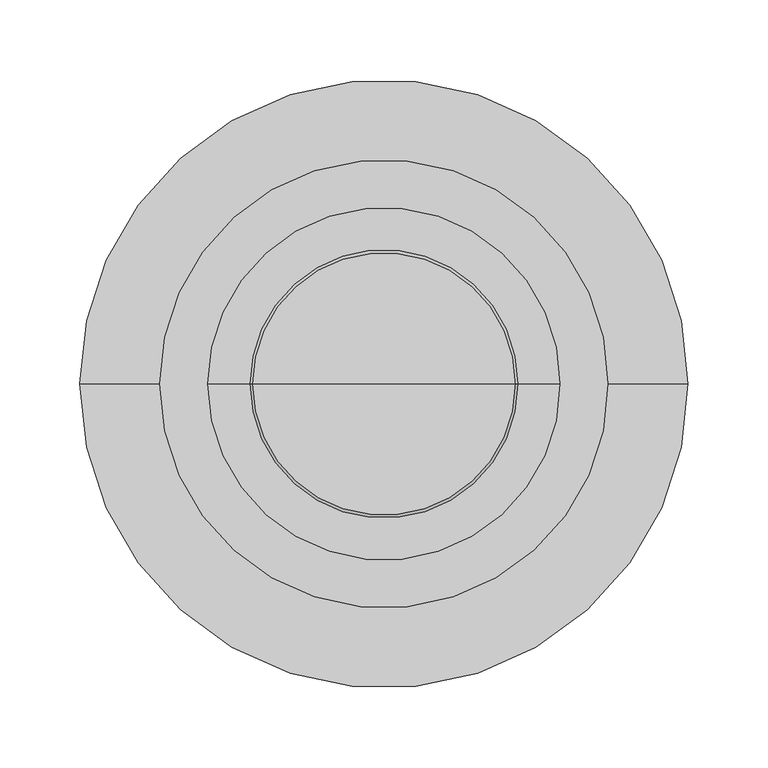
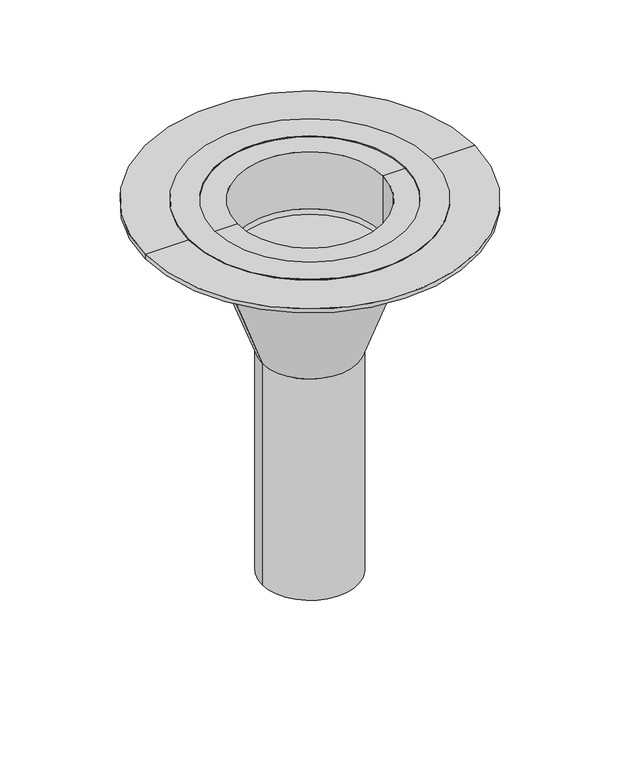
"""IFC4 building model written with IfcOpenShell, lengths in millimetres: proxy geometry, TN_Воронка с обжимным фланцем : Воронка с обжимным металлическим фланцем без обогрева Ø110х450мм."""

from ifc_helpers import new_model, si_unit, point, frame, origin, origin_with_axes, origin_2d, place, context, project, spatial, polyline, circle_curve, trimmed, segment, composite_curve, outline, extrude, source, transform, mapped, element, save
from ifc_brep_helpers import plane_surface, cylinder_surface, revolved_surface, advanced_brep


def specialty_equipment_f296e0ad(model_context):
    return source(origin(), model_context, "Body", "SolidModel", [
        extrude(outline(composite_curve([segment(trimmed(circle_curve(origin_2d(), 140.0), [point((-140.0, 0.0))], [point((140.0, 0.0))], False, "CARTESIAN"), True, "CONTINUOUS"), segment(trimmed(circle_curve(origin_2d(), 140.0), [point((140.0, 0.0))], [point((-140.0, 0.0))], False, "CARTESIAN"), True, "CONTINUOUS")], self_intersect=False), holes=[composite_curve([segment(trimmed(circle_curve(origin_2d(), 110.0556416), [point((-110.0556416, 0.0))], [point((110.0556416, 0.0))], True, "CARTESIAN"), True, "CONTINUOUS"), segment(trimmed(circle_curve(origin_2d(), 110.0556416), [point((110.0556416, 0.0))], [point((-110.0556416, 0.0))], True, "CARTESIAN"), True, "CONTINUOUS")], self_intersect=False)]), origin_with_axes(), (0.0, 0.0, 1.0), 1.0),
        advanced_brep(
        [(0.0, 0.0, -450.0), (-55.0, 0.0, -450.0), (55.0, 0.0, -450.0), (190.0, 0.0, 0.0), (-190.0, 0.0, 0.0), (-83.890873, 0.0, 0.0), (83.890873, 0.0, 0.0), (190.0, 0.0, -5.0), (-190.0, 0.0, -5.0), (93.890873, 0.0, -5.0), (-93.890873, 0.0, -5.0), (55.0, 0.0, -179.9935725), (-55.0, 0.0, -179.9935725), (-93.890873, 0.0, -71.109127), (93.890873, 0.0, -71.109127), (81.9669914, 0.0, -74.7632135), (-81.9669914, 0.0, -74.7632135), (0.0, 0.0, -74.7632135), (83.890873, 0.0, -69.3768397), (-83.890873, 0.0, -69.3768397)],
        [
            (0, 1),
            (1, 2, circle_curve(frame((0.0, 0.0, -450.0), z_axis=(0.0, 0.0, -1.0), x_axis=(-1.0, 0.0, 0.0)), 55.0)),
            (2, 0),
            (2, 1, circle_curve(frame((0.0, 0.0, -450.0), z_axis=(0.0, 0.0, -1.0), x_axis=(-1.0, 0.0, 0.0)), 55.0)),
            (3, 4, circle_curve(frame((0.0, 0.0, 0.0), z_axis=(0.0, 0.0, 1.0), x_axis=(-1.0, 0.0, 0.0)), 190.0)),
            (4, 5),
            (5, 6, circle_curve(frame((0.0, 0.0, 0.0), z_axis=(0.0, 0.0, -1.0), x_axis=(-1.0, 0.0, 0.0)), 83.890873)),
            (6, 3),
            (4, 3, circle_curve(frame((0.0, 0.0, 0.0), z_axis=(0.0, 0.0, 1.0), x_axis=(-1.0, 0.0, 0.0)), 190.0)),
            (6, 5, circle_curve(frame((0.0, 0.0, 0.0), z_axis=(0.0, 0.0, -1.0), x_axis=(-1.0, 0.0, 0.0)), 83.890873)),
            (7, 8, circle_curve(frame((0.0, 0.0, -5.0), z_axis=(0.0, 0.0, 1.0), x_axis=(-1.0, 0.0, 0.0)), 190.0)),
            (8, 4),
            (3, 7),
            (8, 7, circle_curve(frame((0.0, 0.0, -5.0), z_axis=(0.0, 0.0, 1.0), x_axis=(-1.0, 0.0, 0.0)), 190.0)),
            (9, 10, circle_curve(frame((0.0, 0.0, -5.0), z_axis=(0.0, 0.0, 1.0), x_axis=(-1.0, 0.0, 0.0)), 93.890873)),
            (10, 8),
            (7, 9),
            (10, 9, circle_curve(frame((0.0, 0.0, -5.0), z_axis=(0.0, 0.0, 1.0), x_axis=(-1.0, 0.0, 0.0)), 93.890873)),
            (11, 12, circle_curve(frame((0.0, 0.0, -179.9935725), z_axis=(0.0, 0.0, 1.0), x_axis=(-1.0, 0.0, 0.0)), 55.0)),
            (12, 13),
            (13, 14, circle_curve(frame((0.0, 0.0, -71.109127), z_axis=(0.0, 0.0, -1.0), x_axis=(-1.0, 0.0, 0.0)), 93.890873)),
            (14, 11),
            (12, 11, circle_curve(frame((0.0, 0.0, -179.9935725), z_axis=(0.0, 0.0, 1.0), x_axis=(-1.0, 0.0, 0.0)), 55.0)),
            (14, 13, circle_curve(frame((0.0, 0.0, -71.109127), z_axis=(0.0, 0.0, -1.0), x_axis=(-1.0, 0.0, 0.0)), 93.890873)),
            (1, 12),
            (11, 2),
            (15, 16, circle_curve(frame((0.0, 0.0, -74.7632135), z_axis=(0.0, 0.0, 1.0), x_axis=(-1.0, 0.0, 0.0)), 81.9669914)),
            (16, 17),
            (17, 15),
            (16, 15, circle_curve(frame((0.0, 0.0, -74.7632135), z_axis=(0.0, 0.0, 1.0), x_axis=(-1.0, 0.0, 0.0)), 81.9669914)),
            (18, 19, circle_curve(frame((0.0, 0.0, -69.3768397), z_axis=(0.0, 0.0, 1.0), x_axis=(-1.0, 0.0, 0.0)), 83.890873)),
            (19, 16),
            (15, 18),
            (19, 18, circle_curve(frame((0.0, 0.0, -69.3768397), z_axis=(0.0, 0.0, 1.0), x_axis=(-1.0, 0.0, 0.0)), 83.890873)),
            (5, 19),
            (18, 6),
            (13, 10),
            (9, 14),
        ],
        [
            plane_surface(frame((0.0, 0.0, -450.0), z_axis=(0.0, 0.0, -1.0), x_axis=(-1.0, 0.0, 0.0))),
            plane_surface(frame((0.0, 0.0, 0.0), z_axis=(0.0, 0.0, 1.0), x_axis=(-1.0, 0.0, 0.0))),
            cylinder_surface(frame((0.0, 0.0, 0.0), z_axis=(0.0, 0.0, -1.0), x_axis=(-1.0, 0.0, 0.0)), 190.0),
            plane_surface(frame((0.0, 0.0, -5.0), z_axis=(0.0, 0.0, -1.0), x_axis=(-1.0, 0.0, 0.0))),
            revolved_surface(polyline([(-93.890873, 0.0, -71.109127), (-55.0, 0.0, -179.9935725)]), (0.0, 0.0, 0.0), (0.0, 0.0, -1.0)),
            cylinder_surface(frame((0.0, 0.0, 0.0), z_axis=(0.0, 0.0, -1.0), x_axis=(-1.0, 0.0, 0.0)), 55.0),
            plane_surface(frame((0.0, 0.0, -74.7632135), z_axis=(0.0, 0.0, 1.0), x_axis=(-1.0, 0.0, 0.0))),
            revolved_surface(polyline([(-81.9669914, 0.0, -74.7632135), (-83.890873, 0.0, -69.3768397)]), (0.0, 0.0, 0.0), (0.0, 0.0, -1.0)),
            revolved_surface(polyline([(-83.890873, 0.0, -69.3768397), (-83.890873, 0.0, 0.0)]), (0.0, 0.0, 0.0), (0.0, 0.0, -1.0)),
            cylinder_surface(frame((0.0, 0.0, 0.0), z_axis=(0.0, 0.0, -1.0), x_axis=(-1.0, 0.0, 0.0)), 93.890873),
        ],
        [
            (0, [[1, 2, 3]]),
            (0, [[-3, 4, -1]]),
            (1, [[5, 6, 7, 8]]),
            (1, [[9, -8, 10, -6]]),
            (2, [[11, 12, -5, 13]]),
            (2, [[14, -13, -9, -12]]),
            (3, [[15, 16, -11, 17]]),
            (3, [[18, -17, -14, -16]]),
            (4, [[19, 20, 21, 22]]),
            (4, [[23, -22, 24, -20]]),
            (5, [[-2, 25, -19, 26]]),
            (5, [[-4, -26, -23, -25]]),
            (6, [[27, 28, 29]]),
            (6, [[30, -29, -28]]),
            (7, [[31, 32, -27, 33]]),
            (7, [[34, -33, -30, -32]]),
            (8, [[-7, 35, -31, 36]]),
            (8, [[-10, -36, -34, -35]]),
            (9, [[-21, 37, -15, 38]]),
            (9, [[-24, -38, -18, -37]]),
        ],
    ),
    ])


if __name__ == "__main__":
    model = new_model("IFC4")
    model_context = context("Model", 3, world=origin())
    ifc_project = project(units=[si_unit("LENGTHUNIT", "METRE", prefix="MILLI")], contexts=[model_context])
    site = spatial("IfcSite", under=ifc_project)
    building = spatial("IfcBuilding", under=site)
    placement = place(None, origin())
    specialty_equipment_shape = specialty_equipment_f296e0ad(model_context)
    element("IfcBuildingElementProxy", 1, Name="TN_Воронка с обжимным фланцем : Воронка с обжимным металлическим фланцем без обогрева Ø110х450мм", ObjectType="TN_Воронка с обжимным фланцем : Воронка с обжимным металлическим фланцем без обогрева Ø110х450мм", at=placement, inside=building, context=model_context, shape_type="MappedRepresentation", body=[
        mapped(specialty_equipment_shape, transform((0.0, 0.0, 0.0), x_axis=(1.0, 0.0, 0.0), y_axis=(0.0, 1.0, 0.0), z_axis=(0.0, 0.0, 1.0))),
    ])
    save(model, "model.ifc")

# Revit data of these elements
# Type "TN_Воронка с обжимным фланцем : Воронка с обжимным металлическим фланцем без обогрева Ø110х450мм"
#   ADSK_Группирование = "Комплектующие и воронки"
#   Description = "Кровельная воронка с листвоуловителем и обжимным фланцем из нержавеющей стали. Применяется для всех типов гидроизоляционных материалов. Воронка \r\nизготовлена из высокопрочного материала, устойчивого к атмосферному воздействию и ультрафиолетовому излучению. Крепеж- гайка и барашки."
#   Manufacturer = "ТехноНИКОЛЬ"
#   URL = "https://shop.tn.ru/voronka-s-obzhimnym-metallicheskim-flancem-bez-obogreva-o110h450mm"
#   ADSK_Примечание = ""
#   ADSK_Обозначение = "ТехноНИКОЛЬ"
#   ADSK_Наименование = "Воронка с обжимным металлическим фланцем без обогрева Ø110х450мм"
#   ADSK_Масса_Текст = ""
#   ADSK_Марка = ""
#   ADSK_Код изделия = "661125"
#   ADSK_Завод-изготовитель = "ТехноНИКОЛЬ"
#   ADSK_Единица измерения = "шт."
#   ADSK_Группирование = "Комплектующие и воронки"
#   ADSK_URL страницы изделия = "https://shop.tn.ru/voronka-s-obzhimnym-metallicheskim-flancem-bez-obogreva-o110h450mm"
#   ADSK_URL документации изделия = "https://shop.tn.ru/media/other_documents/_661125_661124_661134_671701_671702_661132_661131_661130.pdf"
#   Тип воронки = 1
#   Радиус = 55 mm
#   Пропускная способность = 7.8 L/s
#   Монтажный диаметр = 110 mm
#   Длина расчетная [instance default] = 450 mm
#   Длина отвода [instance default] = 450 mm
#   ADSK_Масса = 2
#   ADSK_Количество = 1
#   Видимость_Листоуловитель [instance default] = yes
#   Материал_Фланец = TN_ПВХ_Серый
#   Материал_Корпус = TN_ПВХ_Черный
#   Default Elevation = 0
# Element 1 (IfcBuildingElementProxy, "TN_Воронка с обжимным фланцем : Воронка с обжимным металлическим фланцем без обогрева Ø110х450мм")
#   Длина отвода = 750 mm
#   Видимость_Листоуловитель = no
#   Materials on its faces: "TN_ПВХ_Черный", "TN_ПВХ_Серый"
# Materials
#   "TN_ПВХ_Серый": class "Типовые", colour RGB 192 192 192, transparency 0, Cost = 0
#   "TN_ПВХ_Черный": class "Типовые", colour RGB 48 48 48, transparency 0, Cost = 0
